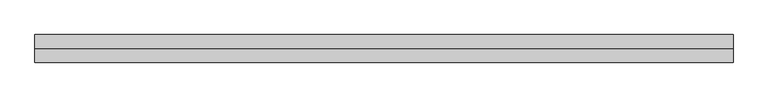
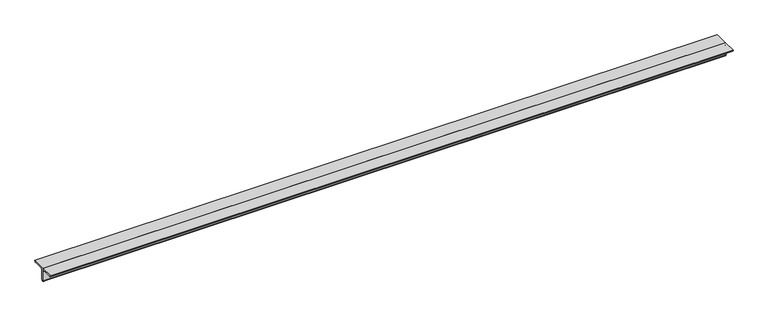
"""IFC4 building model written with IfcOpenShell, lengths in millimetres: beam geometry, 0123_Steel Framing_2Ls-KSD3502 : H_SB_AR_S04_2Ls-130x130x12_VBR1."""

from ifc_helpers import new_model, si_unit, point, frame, frame_2d, origin, place, context, project, spatial, polyline, circle_curve, trimmed, segment, composite_curve, outline, extrude, source, transform, mapped, element, save


def beam_58c1f9d3(model_context):
    return source(origin(), model_context, "Body", "SweptSolid", [
        extrude(outline(composite_curve([segment(polyline([(0.0, 36.4), (130.0, 36.4)]), True, "CONTINUOUS"), segment(trimmed(circle_curve(frame_2d((118.0, 36.4)), 12.0), [point((130.0, 36.4))], [point((118.0, 24.4))], False, "CARTESIAN"), True, "CONTINUOUS"), segment(polyline([(118.0, 24.4), (24.0, 24.4)]), True, "CONTINUOUS"), segment(trimmed(circle_curve(frame_2d((24.0, 12.4)), 12.0), [point((24.0, 24.4))], [point((12.0, 12.4))], True, "CARTESIAN"), True, "CONTINUOUS"), segment(polyline([(12.0, 12.4), (12.0, -81.6)]), True, "CONTINUOUS"), segment(trimmed(circle_curve(frame_2d((0.0, -81.6)), 12.0), [point((12.0, -81.6))], [point((0.0, -93.6))], False, "CARTESIAN"), True, "CONTINUOUS"), segment(polyline([(0.0, -93.6), (0.0, 36.4)]), True, "CONTINUOUS")], self_intersect=False)), frame((-3283.9548965, 0.0, 0.0), z_axis=(1.0, 0.0, 0.0), x_axis=(0.0, 1.0, 0.0)), (0.0, 0.0, 1.0), 6570.1314861),
        extrude(outline(composite_curve([segment(polyline([(0.0, 36.4), (0.0, -93.6)]), True, "CONTINUOUS"), segment(trimmed(circle_curve(frame_2d((0.0, -81.6)), 12.0), [point((0.0, -93.6))], [point((-12.0, -81.6))], False, "CARTESIAN"), True, "CONTINUOUS"), segment(polyline([(-12.0, -81.6), (-12.0, 12.4)]), True, "CONTINUOUS"), segment(trimmed(circle_curve(frame_2d((-24.0, 12.4)), 12.0), [point((-12.0, 12.4))], [point((-24.0, 24.4))], True, "CARTESIAN"), True, "CONTINUOUS"), segment(polyline([(-24.0, 24.4), (-118.0, 24.4)]), True, "CONTINUOUS"), segment(trimmed(circle_curve(frame_2d((-118.0, 36.4)), 12.0), [point((-118.0, 24.4))], [point((-130.0, 36.4))], False, "CARTESIAN"), True, "CONTINUOUS"), segment(polyline([(-130.0, 36.4), (0.0, 36.4)]), True, "CONTINUOUS")], self_intersect=False)), frame((-3283.9548965, 0.0, 0.0), z_axis=(1.0, 0.0, 0.0), x_axis=(0.0, 1.0, 0.0)), (0.0, 0.0, 1.0), 6570.1314861),
    ])


if __name__ == "__main__":
    model = new_model("IFC4")
    model_context = context("Model", 3, world=origin())
    ifc_project = project(units=[si_unit("LENGTHUNIT", "METRE", prefix="MILLI")], contexts=[model_context])
    site = spatial("IfcSite", under=ifc_project)
    building = spatial("IfcBuilding", under=site)
    placement = place(None, origin())
    beam_shape = beam_58c1f9d3(model_context)
    element("IfcBeam", 1, ObjectType="0123_Steel Framing_2Ls-KSD3502 : H_SB_AR_S04_2Ls-130x130x12_VBR1", at=placement, inside=building, context=model_context, shape_type="MappedRepresentation", body=[
        mapped(beam_shape, transform((0.0, 0.0, 0.0), x_axis=(1.0, 0.0, 0.0), y_axis=(0.0, 1.0, 0.0), z_axis=(0.0, 0.0, 1.0))),
    ])
    save(model, "model.ifc")

# Revit data of these elements
# Type "0123_Steel Framing_2Ls-KSD3502 : H_SB_AR_S04_2Ls-130x130x12_VBR1"
#   Type Mark = "VBR1"
#   Assembly Code = "B10"
#   Legs = "SLBB"
#   W = 8.97
#   Perimeter = 1.04 m²/m
#   Nominal Weight = 46.80 kgf/m
#   Length [instance default] = 1000 mm
#   Space = 0 mm
#   b = 130 mm
#   d = 130 mm
#   t = 12 mm
#   y = 36.4 mm
#   A = 0.005952 m²
#   Structural Material [instance default] = Steel ASTM A36
# Element 1 (IfcBeam, "0123_Steel Framing_2Ls-KSD3502 : H_SB_AR_S04_2Ls-130x130x12_VBR1")
#   Materials on its faces: "Steel ASTM A36"
# Materials
#   "Steel ASTM A36": class "Metal", colour RGB 199 199 199, transparency 0, Description = "Structural steel, ASTM A36 Grade B, mill finish", Cost = 0
